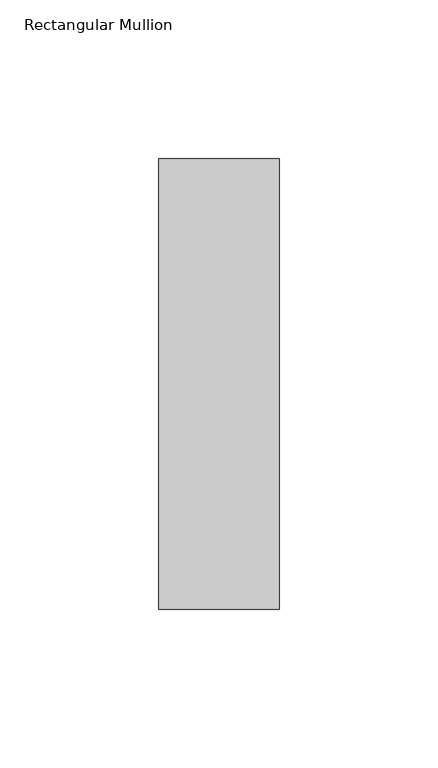
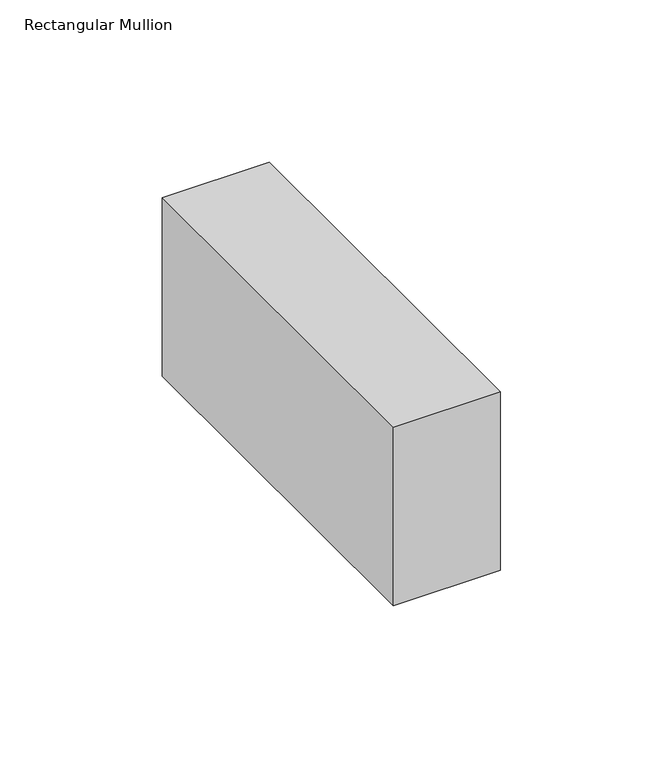
"""IFC4 building model written with IfcOpenShell, lengths in millimetres: member geometry, Rectangular Mullion : NLRS_21_CWM_hsb-regel 38x142_gen_rsf."""

from ifc_helpers import new_model, si_unit, frame, origin, place, context, project, spatial, polyline, outline, extrude, source, transform, mapped, element, save


def rectangular_mullion_8284db35(model_context):
    return source(origin(), model_context, "Body", "SweptSolid", [
        extrude(outline(polyline([(-38.0, -71.0), (-38.0, 71.0), (0.0, 71.0), (0.0, -71.0), (-38.0, -71.0)])), frame((0.0, 0.0, -66.9999997), z_axis=(0.0, 0.0, 1.0), x_axis=(1.0, 0.0, 0.0)), (0.0, 0.0, 1.0), 66.9999997),
    ])


if __name__ == "__main__":
    model = new_model("IFC4")
    model_context = context("Model", 3, world=origin())
    ifc_project = project(units=[si_unit("LENGTHUNIT", "METRE", prefix="MILLI")], contexts=[model_context])
    site = spatial("IfcSite", under=ifc_project)
    building = spatial("IfcBuilding", under=site)
    placement = place(None, origin())
    rectangular_mullion_shape = rectangular_mullion_8284db35(model_context)
    element("IfcMember", 1, ObjectType="Rectangular Mullion : NLRS_21_CWM_hsb-regel 38x142_gen_rsf", at=placement, inside=building, context=model_context, shape_type="MappedRepresentation", body=[
        mapped(rectangular_mullion_shape, transform((0.0, 0.0, 0.0), x_axis=(1.0, 0.0, 0.0), y_axis=(0.0, 1.0, 0.0), z_axis=(0.0, 0.0, 1.0))),
    ])
    save(model, "model.ifc")

# Revit data of these elements
# Type "Rectangular Mullion : NLRS_21_CWM_hsb-regel 38x142_gen_rsf"
#   Export Type to IFC As = "IfcWall"
#   Type IfcGUID = "07M7mRoiH1CR8m_RSKIwpF"
#   Assembly Code = "21.10"
#   built-in parameter 1007322 = 0.465879 (stored number, unit not read)
#   built-in parameter 1007321 = 0.062336 (stored number, unit not read)
#   built-in parameter 1007320 = 0.062336 (stored number, unit not read)
# Element 1 (IfcMember, "Rectangular Mullion : NLRS_21_CWM_hsb-regel 38x142_gen_rsf")
#   Materials on its faces: "NLRS_i2_hout naaldhout vuren_gen_rsf"
# Materials
#   "NLRS_i2_hout naaldhout vuren_gen_rsf": class "I - Hout", colour RGB 234 199 147, transparency 0, Keynote = "i2", Manufacturer = "Revit Standards Foundation", URL = "www.revitstandards.org", Description = "hout vuren", Cost = 0
